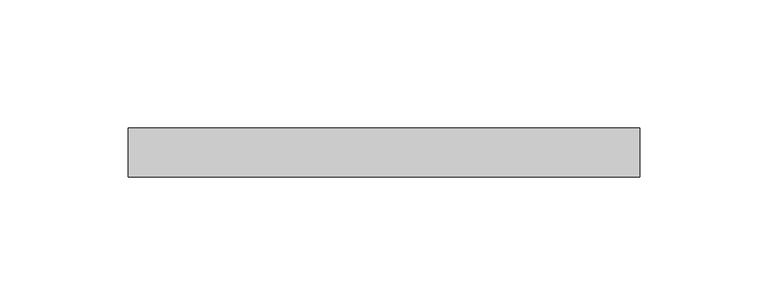
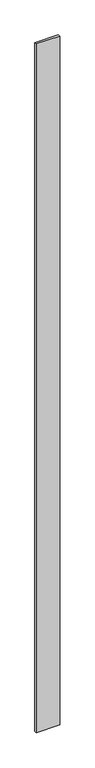
"""IFC4 building model written with IfcOpenShell, lengths in millimetres: proxy geometry, Inner panel:Inner panel:1:Inner panel:1 : Inner panel:Inner panel:300324:300043:Inner panel:1:Inner panel:1 : Inner panel:Inner panel:300324:300043 : Inner panel:Inner panel:1:Inner panel:1 : Inner panel:Inner panel:300324:300043:41 : Inner panel:Inner panel:1:Inner panel:1 : Inner panel:Inner panel:300324:300043:Inner panel:1:Inner panel:1 : Inner panel:Inner panel:300324:300043 : Inner panel:Inner panel:1:Inner panel:1 : Inner panel:Inner panel:300324:300043:300031."""

from ifc_helpers import new_model, si_unit, origin, origin_with_axes, place, context, project, spatial, polyline, outline, extrude, source, transform, mapped, element, save


def generic_models_07a0c0ad(model_context):
    return source(origin(), model_context, "Body", "SweptSolid", [
        extrude(outline(polyline([(667344.1117239, -568187.237148), (667543.2495663, -568187.237148), (667543.2495663, -568206.287148), (667344.1117239, -568206.287148), (667344.1117239, -568187.237148)])), origin_with_axes(), (0.0, 0.0, 1.0), 6165.85),
    ])


if __name__ == "__main__":
    model = new_model("IFC4")
    model_context = context("Model", 3, world=origin())
    ifc_project = project(units=[si_unit("LENGTHUNIT", "METRE", prefix="MILLI")], contexts=[model_context])
    site = spatial("IfcSite", under=ifc_project)
    building = spatial("IfcBuilding", under=site)
    placement = place(None, origin())
    generic_models_shape = generic_models_07a0c0ad(model_context)
    element("IfcBuildingElementProxy", 1, Name="Inner panel:Inner panel:1:Inner panel:1 : Inner panel:Inner panel:300324:300043:Inner panel:1:Inner panel:1 : Inner panel:Inner panel:300324:300043 : Inner panel:Inner panel:1:Inner panel:1 : Inner panel:Inner panel:300324:300043:41 : Inner panel:Inner panel:1:Inner panel:1 : Inner panel:Inner panel:300324:300043:Inner panel:1:Inner panel:1 : Inner panel:Inner panel:300324:300043 : Inner panel:Inner panel:1:Inner panel:1 : Inner panel:Inner panel:300324:300043:300031", ObjectType="Inner panel:Inner panel:1:Inner panel:1 : Inner panel:Inner panel:300324:300043:Inner panel:1:Inner panel:1 : Inner panel:Inner panel:300324:300043 : Inner panel:Inner panel:1:Inner panel:1 : Inner panel:Inner panel:300324:300043:41 : Inner panel:Inner panel:1:Inner panel:1 : Inner panel:Inner panel:300324:300043:Inner panel:1:Inner panel:1 : Inner panel:Inner panel:300324:300043 : Inner panel:Inner panel:1:Inner panel:1 : Inner panel:Inner panel:300324:300043:300031", at=placement, inside=building, context=model_context, shape_type="MappedRepresentation", body=[
        mapped(generic_models_shape, transform((0.0, 0.0, 0.0), x_axis=(1.0, 0.0, 0.0), y_axis=(0.0, 1.0, 0.0), z_axis=(0.0, 0.0, 1.0))),
    ])
    save(model, "model.ifc")

# Revit data of these elements
# Type "Inner panel:Inner panel:1:Inner panel:1 : Inner panel:Inner panel:300324:300043:Inner panel:1:Inner panel:1 : Inner panel:Inner panel:300324:300043 : Inner panel:Inner panel:1:Inner panel:1 : Inner panel:Inner panel:300324:300043:41 : Inner panel:Inner panel:1:Inner panel:1 : Inner panel:Inner panel:300324:300043:Inner panel:1:Inner panel:1 : Inner panel:Inner panel:300324:300043 : Inner panel:Inner panel:1:Inner panel:1 : Inner panel:Inner panel:300324:300043:300031"
#   NameOverride = "Inner panel:Inner panel:1:Inner panel:1 : Inner panel:Inner panel:300324:300043:Inner panel:1:Inner panel:1 : Inner panel:Inner panel:300324:300043 : Inner panel:Inner panel:1:Inner panel:1 : Inner panel:Inner panel:300324:300043:300031"
#   ObjectTypeOverride = "Inner panel:1:Inner panel:1 : Inner panel:Inner panel:300324:300043 : Inner panel:Inner panel:1:Inner panel:1 : Inner panel:Inner panel:300324:300043"
#   Reference = "Inner panel"
#   Tag = "300031"
# Element 1 (IfcBuildingElementProxy, "Inner panel:Inner panel:1:Inner panel:1 : Inner panel:Inner panel:300324:300043:Inner panel:1:Inner panel:1 : Inner panel:Inner panel:300324:300043 : Inner panel:Inner panel:1:Inner panel:1 : Inner panel:Inner panel:300324:300043:41 : Inner panel:Inner panel:1:Inner panel:1 : Inner panel:Inner panel:300324:300043:Inner panel:1:Inner panel:1 : Inner panel:Inner panel:300324:300043 : Inner panel:Inner panel:1:Inner panel:1 : Inner panel:Inner panel:300324:300043:300031")
#   Materials on its faces: "¾” (CLASS A) FIRE RETARDANT PLYWOOD ...OR… IF 1/4\" GYP. BD UNDER PLYWOOD, FLAME SPREAD TO BE CLASS B -  (FINISH: GRADE B - PREFINISHED STAINED/SEALED) - 1/4\" GAP BTWN PANELS (FASTENERS T.B.D.)"
# Materials
#   "¾” (CLASS A) FIRE RETARDANT PLYWOOD ...OR… IF 1/4\" GYP. BD UNDER PLYWOOD, FLAME SPREAD TO BE CLASS B -  (FINISH: GRADE B - PREFINISHED STAINED/SEALED) - 1/4\" GAP BTWN PANELS (FASTENERS T.B.D.)": class "Wood", colour RGB 149 120 74, transparency 0, Description = "Plywood, sheathing grade", Cost = 0
